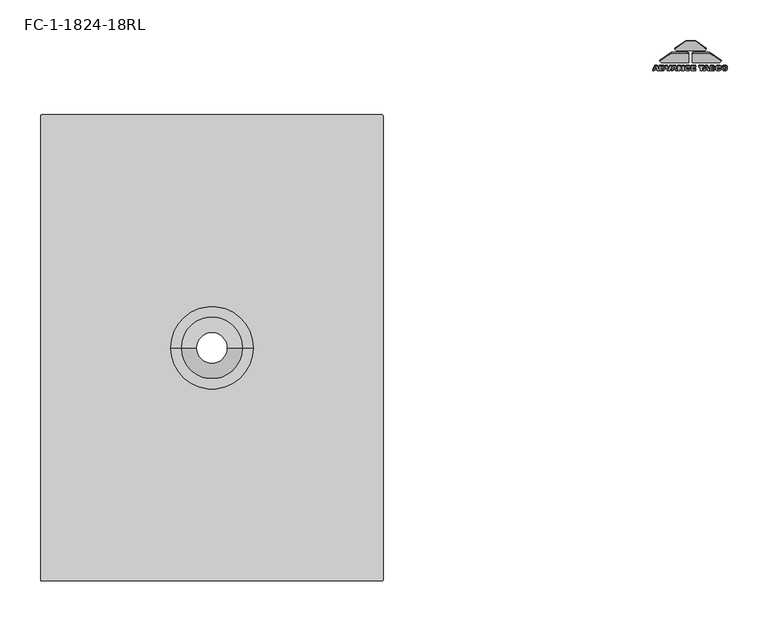
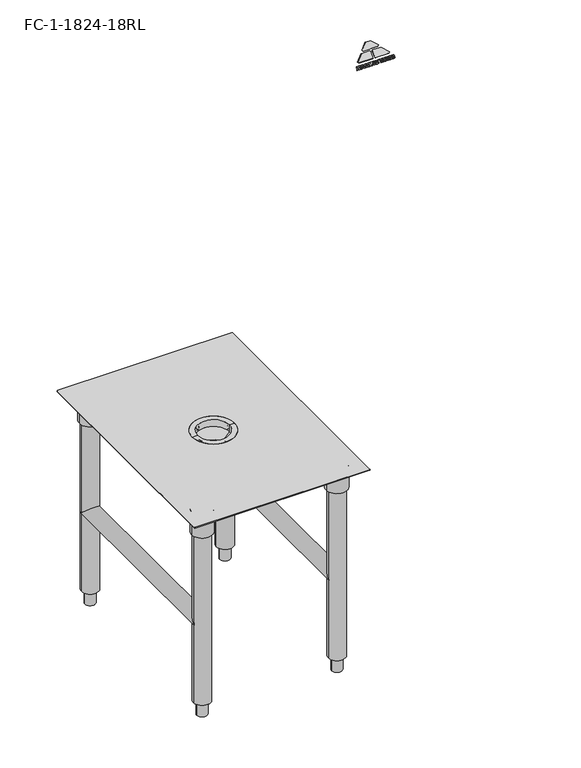
"""IFC4 building model written with IfcOpenShell, lengths in millimetres: proxy geometry, qf_advance_fc-1$2014$FC-1-1824-18RL : FC-1-1824-18RL."""

from ifc_helpers import new_model, si_unit, point, frame, frame_2d, origin, origin_with_axes, place, context, project, spatial, polyline, circle_curve, trimmed, segment, composite_curve, outline, extrude, source, transform, mapped, element, save
from ifc_brep_helpers import plane_surface, cylinder_surface, revolved_surface, advanced_brep


def fc_1_1824_18rl_d9c02636(model_context):
    return source(origin(), model_context, "Body", "SolidModel", [
        extrude(outline(polyline([(0.0, 0.0), (0.8986382, -2.992169), (-5.7928564, -7.4682591), (-6.3992546, -5.4491532), (-5.2268421, -4.6727099), (-6.0231962, -2.021113), (-7.4220948, -2.0434324), (-8.0357989, 0.0), (0.0, 0.0)]), holes=[polyline([(-1.0236432, -1.9782405), (-4.4880528, -2.0109168), (-3.9335816, -3.857123), (-1.0236432, -1.9782405)])]), frame((1231.0364, -35.8439941, 1043.6560059), z_axis=(0.0, -0.7071067811865482, 0.7071067811865468), x_axis=(0.28763785914895384, 0.6772239149587841, 0.6772239149587854)), (0.0, 0.0, 1.0), 1.5875),
        extrude(outline(composite_curve([segment(polyline([(1.7388284, -5.7897253), (2.9132681, -9.7002225)]), True, "CONTINUOUS"), segment(trimmed(circle_curve(frame_2d((0.4258756, -10.4472612)), 2.59715), [point((2.9132681, -9.7002225))], [point((1.1729143, -12.9346537))], False, "CARTESIAN"), True, "CONTINUOUS"), segment(polyline([(1.1729143, -12.9346537), (-1.2232536, -13.6542948)]), True, "CONTINUOUS"), segment(trimmed(circle_curve(frame_2d((-1.9702922, -11.1669024)), 2.59715), [point((-1.2232536, -13.6542948))], [point((-4.4576846, -11.913941))], False, "CARTESIAN"), True, "CONTINUOUS"), segment(polyline([(-4.4576846, -11.913941), (-5.6321244, -8.0034438), (1.7388284, -5.7897253)]), True, "CONTINUOUS")], self_intersect=False), holes=[composite_curve([segment(polyline([(-3.3131514, -9.4551704), (-2.7304978, -11.3952149)]), True, "CONTINUOUS"), segment(trimmed(circle_curve(frame_2d((-1.9702922, -11.1669024)), 0.79375), [point((-2.7304978, -11.3952149))], [point((-1.7419797, -11.9271079))], True, "CARTESIAN"), True, "CONTINUOUS"), segment(polyline([(-1.7419797, -11.9271079), (0.6541882, -11.2074667)]), True, "CONTINUOUS"), segment(trimmed(circle_curve(frame_2d((0.4258756, -10.4472612)), 0.79375), [point((0.6541882, -11.2074667))], [point((1.1860812, -10.2189486))], True, "CARTESIAN"), True, "CONTINUOUS"), segment(polyline([(1.1860812, -10.2189486), (0.6034275, -8.2789041), (-3.3131514, -9.4551704)]), True, "CONTINUOUS")], self_intersect=False)]), frame((1231.0364, -35.8439941, 1043.6560059), z_axis=(0.0, -0.7071067811865482, 0.7071067811865468), x_axis=(0.28763785914895384, 0.6772239149587841, 0.6772239149587854)), (0.0, 0.0, 1.0), 1.5875),
        extrude(outline(polyline([(3.8502629, -12.820106), (4.449355, -14.8148853), (-0.7608679, -18.1300438), (5.4356652, -18.0989732), (6.0493693, -20.1424056), (-1.9718176, -20.1910588), (-2.8923738, -17.1259101), (3.8502629, -12.820106)])), frame((1231.0364, -35.8439941, 1043.6560059), z_axis=(0.0, -0.7071067811865482, 0.7071067811865468), x_axis=(0.28763785914895384, 0.6772239149587841, 0.6772239149587854)), (0.0, 0.0, 1.0), 1.5875),
        extrude(outline(polyline([(-0.8905293, -23.7913921), (-1.5042335, -21.7479597), (6.5315655, -21.7479597), (7.4302036, -24.7401286), (0.738709, -29.2162188), (0.1323109, -27.1971129), (1.3047234, -26.4206696), (0.5083692, -23.7690727), (-0.8905293, -23.7913921)]), holes=[polyline([(2.0435127, -23.7588764), (2.5979839, -25.6050827), (5.5079223, -23.7262001), (2.0435127, -23.7588764)])]), frame((1231.0364, -35.8439941, 1043.6560059), z_axis=(0.0, -0.7071067811865482, 0.7071067811865468), x_axis=(0.28763785914895384, 0.6772239149587841, 0.6772239149587854)), (0.0, 0.0, 1.0), 1.5875),
        extrude(outline(polyline([(0.8994411, -29.7514035), (8.2703938, -27.537685), (9.2640101, -30.8460994), (4.2655808, -34.6015449), (9.8850202, -32.9138585), (10.4768063, -34.8843112), (3.1058536, -37.0980297), (2.0976253, -33.7409621), (7.1447075, -29.9709047), (1.4766152, -31.673203), (0.8994411, -29.7514035)])), frame((1231.0364, -35.8439941, 1043.6560059), z_axis=(0.0, -0.7071067811865482, 0.7071067811865468), x_axis=(0.28763785914895384, 0.6772239149587841, 0.6772239149587854)), (0.0, 0.0, 1.0), 1.5875),
        extrude(outline(composite_curve([segment(polyline([(10.2323563, -43.0996089), (9.7136302, -41.372422)]), True, "CONTINUOUS"), segment(trimmed(circle_curve(frame_2d((9.4853176, -40.6122165)), 0.79375), [point((9.7136302, -41.372422))], [point((10.2455232, -40.3839039))], True, "CARTESIAN"), True, "CONTINUOUS"), segment(polyline([(10.2455232, -40.3839039), (9.7888981, -38.8634929)]), True, "CONTINUOUS"), segment(trimmed(circle_curve(frame_2d((9.0286925, -39.0918054)), 0.79375), [point((9.7888981, -38.8634929))], [point((8.80038, -38.3315999))], True, "CARTESIAN"), True, "CONTINUOUS"), segment(polyline([(8.80038, -38.3315999), (6.4042121, -39.0512411)]), True, "CONTINUOUS"), segment(trimmed(circle_curve(frame_2d((6.6325247, -39.8114466)), 0.79375), [point((6.4042121, -39.0512411))], [point((5.8723192, -40.0397591))], True, "CARTESIAN"), True, "CONTINUOUS"), segment(polyline([(5.8723192, -40.0397591), (6.3289443, -41.5601702)]), True, "CONTINUOUS"), segment(trimmed(circle_curve(frame_2d((7.0891498, -41.3318576)), 0.79375), [point((6.3289443, -41.5601702))], [point((7.3174623, -42.0920632))], True, "CARTESIAN"), True, "CONTINUOUS"), segment(polyline([(7.3174623, -42.0920632), (7.8361884, -43.8192501)]), True, "CONTINUOUS"), segment(trimmed(circle_curve(frame_2d((7.0891498, -41.3318576)), 2.59715), [point((7.8361884, -43.8192501))], [point((4.6017574, -42.0788963))], False, "CARTESIAN"), True, "CONTINUOUS"), segment(polyline([(4.6017574, -42.0788963), (4.1451323, -40.5584852)]), True, "CONTINUOUS"), segment(trimmed(circle_curve(frame_2d((6.6325247, -39.8114466)), 2.59715), [point((4.1451323, -40.5584852))], [point((5.885486, -37.3240541))], False, "CARTESIAN"), True, "CONTINUOUS"), segment(polyline([(5.885486, -37.3240541), (8.2816539, -36.6044129)]), True, "CONTINUOUS"), segment(trimmed(circle_curve(frame_2d((9.0286925, -39.0918054)), 2.59715), [point((8.2816539, -36.6044129))], [point((11.5160851, -38.3447667))], False, "CARTESIAN"), True, "CONTINUOUS"), segment(polyline([(11.5160851, -38.3447667), (11.9727102, -39.8651778)]), True, "CONTINUOUS"), segment(trimmed(circle_curve(frame_2d((9.4853176, -40.6122165)), 2.59715), [point((11.9727102, -39.8651778))], [point((10.2323563, -43.0996089))], False, "CARTESIAN"), True, "CONTINUOUS")], self_intersect=False)), frame((1231.0364, -35.8439941, 1043.6560059), z_axis=(0.0, -0.7071067811865482, 0.7071067811865468), x_axis=(0.28763785914895384, 0.6772239149587841, 0.6772239149587854)), (0.0, 0.0, 1.0), 1.5875),
        extrude(outline(polyline([(12.9681529, -43.1796739), (14.5681672, -48.5071942), (12.9382866, -48.9966963), (11.9300584, -45.6396287), (10.6164232, -46.0341528), (11.5588974, -49.1722812), (10.1722825, -49.5887233), (9.2298083, -46.4505949), (7.8431934, -46.867037), (8.8733397, -50.2970843), (7.2191325, -50.7938924), (5.5972001, -45.3933924), (12.9681529, -43.1796739)])), frame((1231.0364, -35.8439941, 1043.6560059), z_axis=(0.0, -0.7071067811865482, 0.7071067811865468), x_axis=(0.28763785914895384, 0.6772239149587841, 0.6772239149587854)), (0.0, 0.0, 1.0), 1.5875),
        extrude(outline(polyline([(15.6567615, -52.1318541), (17.4102019, -57.9702326), (15.7073414, -58.4816527), (15.1155553, -56.5112), (9.447463, -58.2134984), (8.8556768, -56.2430456), (14.5237692, -54.5407473), (13.953901, -52.6432743), (15.6567615, -52.1318541)])), frame((1231.0364, -35.8439941, 1043.6560059), z_axis=(0.0, -0.7071067811865482, 0.7071067811865468), x_axis=(0.28763785914895384, 0.6772239149587841, 0.6772239149587854)), (0.0, 0.0, 1.0), 1.5875),
        extrude(outline(polyline([(9.9077411, -59.7460727), (17.94354, -59.7460727), (18.8421782, -62.7382416), (12.1506836, -67.2143318), (11.5442854, -65.1952259), (12.7166979, -64.4187826), (11.9203437, -61.7671857), (10.5214452, -61.7895051), (9.9077411, -59.7460727)]), holes=[polyline([(14.0099584, -63.6031957), (16.9198968, -61.7243132), (13.4554872, -61.7569894), (14.0099584, -63.6031957)])]), frame((1231.0364, -35.8439941, 1043.6560059), z_axis=(0.0, -0.7071067811865482, 0.7071067811865468), x_axis=(0.28763785914895384, 0.6772239149587841, 0.6772239149587854)), (0.0, 0.0, 1.0), 1.5875),
        extrude(outline(composite_curve([segment(polyline([(19.6750624, -65.5114714), (20.8732466, -69.50103)]), True, "CONTINUOUS"), segment(trimmed(circle_curve(frame_2d((18.9043499, -69.6343934)), 1.9734082), [point((20.8732466, -69.50103))], [point((17.1877703, -70.6078892))], False, "CARTESIAN"), True, "CONTINUOUS"), segment(trimmed(circle_curve(frame_2d((15.3204157, -71.0793546)), 1.9259524), [point((17.1877703, -70.6078892))], [point((13.4530612, -71.5508198))], False, "CARTESIAN"), True, "CONTINUOUS"), segment(polyline([(13.4530612, -71.5508198), (12.3041096, -67.7251899), (19.6750624, -65.5114714)]), True, "CONTINUOUS")], self_intersect=False), holes=[composite_curve([segment(polyline([(15.6697513, -68.8625705), (14.1644846, -69.3146473), (14.7343527, -71.2121203)]), True, "CONTINUOUS"), segment(trimmed(circle_curve(frame_2d((15.389333, -70.7098113)), 0.8254172), [point((14.7343527, -71.2121203))], [point((16.2133035, -70.6609635))], True, "CARTESIAN"), True, "CONTINUOUS"), segment(polyline([(16.2133035, -70.6609635), (15.6697513, -68.8625705)]), True, "CONTINUOUS")], self_intersect=False), composite_curve([segment(polyline([(18.8038562, -67.9213047), (17.3233327, -68.3659503), (17.8128348, -69.995831)]), True, "CONTINUOUS"), segment(trimmed(circle_curve(frame_2d((18.4548879, -69.4790507)), 0.824193), [point((17.8128348, -69.995831))], [point((19.2787463, -69.5025322))], True, "CARTESIAN"), True, "CONTINUOUS"), segment(polyline([(19.2787463, -69.5025322), (18.8038562, -67.9213047)]), True, "CONTINUOUS")], self_intersect=False)]), frame((1231.0364, -35.8439941, 1043.6560059), z_axis=(0.0, -0.7071067811865482, 0.7071067811865468), x_axis=(0.28763785914895384, 0.6772239149587841, 0.6772239149587854)), (0.0, 0.0, 1.0), 1.5875),
        extrude(outline(composite_curve([segment(trimmed(circle_curve(frame_2d((20.3799312, -76.8876879)), 2.59715), [point((22.8673237, -76.1406493))], [point((21.1269699, -79.3750804))], False, "CARTESIAN"), True, "CONTINUOUS"), segment(polyline([(21.1269699, -79.3750804), (20.6082437, -77.6478935)]), True, "CONTINUOUS"), segment(trimmed(circle_curve(frame_2d((20.3799312, -76.8876879)), 0.79375), [point((20.6082437, -77.6478935))], [point((21.1401367, -76.6593754))], True, "CARTESIAN"), True, "CONTINUOUS"), segment(polyline([(21.1401367, -76.6593754), (20.6835116, -75.1389643)]), True, "CONTINUOUS"), segment(trimmed(circle_curve(frame_2d((19.9233061, -75.3672769)), 0.79375), [point((20.6835116, -75.1389643))], [point((19.6949935, -74.6070714))], True, "CARTESIAN"), True, "CONTINUOUS"), segment(polyline([(19.6949935, -74.6070714), (17.2988257, -75.3267125)]), True, "CONTINUOUS"), segment(trimmed(circle_curve(frame_2d((17.5271382, -76.0869181)), 0.79375), [point((17.2988257, -75.3267125))], [point((16.7669327, -76.3152306))], True, "CARTESIAN"), True, "CONTINUOUS"), segment(polyline([(16.7669327, -76.3152306), (17.2235578, -77.8356417)]), True, "CONTINUOUS"), segment(trimmed(circle_curve(frame_2d((17.9837633, -77.6073291)), 0.79375), [point((17.2235578, -77.8356417))], [point((18.2120759, -78.3675346))], True, "CARTESIAN"), True, "CONTINUOUS"), segment(polyline([(18.2120759, -78.3675346), (18.730802, -80.0947216)]), True, "CONTINUOUS"), segment(trimmed(circle_curve(frame_2d((17.9837633, -77.6073291)), 2.59715), [point((18.730802, -80.0947216))], [point((15.4963709, -78.3543678))], False, "CARTESIAN"), True, "CONTINUOUS"), segment(polyline([(15.4963709, -78.3543678), (15.0397458, -76.8339567)]), True, "CONTINUOUS"), segment(trimmed(circle_curve(frame_2d((17.5271382, -76.0869181)), 2.59715), [point((15.0397458, -76.8339567))], [point((16.7800995, -73.5995256))], False, "CARTESIAN"), True, "CONTINUOUS"), segment(polyline([(16.7800995, -73.5995256), (19.1762674, -72.8798844)]), True, "CONTINUOUS"), segment(trimmed(circle_curve(frame_2d((19.9233061, -75.3672769)), 2.59715), [point((19.1762674, -72.8798844))], [point((22.4106986, -74.6202382))], False, "CARTESIAN"), True, "CONTINUOUS"), segment(polyline([(22.4106986, -74.6202382), (22.8673237, -76.1406493)]), True, "CONTINUOUS")], self_intersect=False)), frame((1231.0364, -35.8439941, 1043.6560059), z_axis=(0.0, -0.7071067811865482, 0.7071067811865468), x_axis=(0.28763785914895384, 0.6772239149587841, 0.6772239149587854)), (0.0, 0.0, 1.0), 1.5875),
        extrude(outline(composite_curve([segment(polyline([(18.9878987, -80.9507689), (21.3840666, -80.2311277)]), True, "CONTINUOUS"), segment(trimmed(circle_curve(frame_2d((22.1311052, -82.7185202)), 2.59715), [point((21.3840666, -80.2311277))], [point((24.6184977, -81.9714815))], False, "CARTESIAN"), True, "CONTINUOUS"), segment(polyline([(24.6184977, -81.9714815), (25.0751228, -83.4918925)]), True, "CONTINUOUS"), segment(trimmed(circle_curve(frame_2d((22.5877303, -84.2389312)), 2.59715), [point((25.0751228, -83.4918925))], [point((23.1187153, -86.7812222))], False, "CARTESIAN"), True, "CONTINUOUS"), segment(polyline([(23.1187153, -86.7812222), (20.7225475, -87.5008633)]), True, "CONTINUOUS"), segment(trimmed(circle_curve(frame_2d((20.1915625, -84.9585724)), 2.59715), [point((20.7225475, -87.5008633))], [point((17.7041701, -85.705611))], False, "CARTESIAN"), True, "CONTINUOUS"), segment(polyline([(17.7041701, -85.705611), (17.247545, -84.1852)]), True, "CONTINUOUS"), segment(trimmed(circle_curve(frame_2d((19.7349374, -83.4381613)), 2.59715), [point((17.247545, -84.1852))], [point((18.9878987, -80.9507689))], False, "CARTESIAN"), True, "CONTINUOUS")], self_intersect=False), holes=[composite_curve([segment(polyline([(18.9747318, -83.6664739), (19.4313569, -85.1868849)]), True, "CONTINUOUS"), segment(trimmed(circle_curve(frame_2d((20.1915625, -84.9585724)), 0.79375), [point((19.4313569, -85.1868849))], [point((20.2994506, -85.7449561))], True, "CARTESIAN"), True, "CONTINUOUS"), segment(polyline([(20.2994506, -85.7449561), (22.6956183, -85.0253149)]), True, "CONTINUOUS"), segment(trimmed(circle_curve(frame_2d((22.5877303, -84.2389312)), 0.79375), [point((22.6956183, -85.0253149))], [point((23.3479358, -84.0106187))], True, "CARTESIAN"), True, "CONTINUOUS"), segment(polyline([(23.3479358, -84.0106187), (22.8913107, -82.4902076)]), True, "CONTINUOUS"), segment(trimmed(circle_curve(frame_2d((22.1311052, -82.7185202)), 0.79375), [point((22.8913107, -82.4902076))], [point((21.9027927, -81.9583146))], True, "CARTESIAN"), True, "CONTINUOUS"), segment(polyline([(21.9027927, -81.9583146), (19.5066248, -82.6779558)]), True, "CONTINUOUS"), segment(trimmed(circle_curve(frame_2d((19.7349374, -83.4381613)), 0.79375), [point((19.5066248, -82.6779558))], [point((18.9747318, -83.6664739))], True, "CARTESIAN"), True, "CONTINUOUS")], self_intersect=False)]), frame((1231.0364, -35.8439941, 1043.6560059), z_axis=(0.0, -0.7071067811865482, 0.7071067811865468), x_axis=(0.28763785914895384, 0.6772239149587841, 0.6772239149587854)), (0.0, 0.0, 1.0), 1.5875),
        extrude(outline(polyline([(55.8503682, -36.1089094), (46.7199535, -52.7744612), (43.69559, -51.7997924), (33.5402477, -17.9858506), (35.527159, -15.5061455), (52.3580994, -24.4808057), (55.8503682, -36.1089094)])), frame((1231.0364, -35.8439941, 1043.6560059), z_axis=(0.0, -0.7071067811865482, 0.7071067811865468), x_axis=(0.28763785914895384, 0.6772239149587841, 0.6772239149587854)), (0.0, 0.0, 1.0), 1.5875),
        extrude(outline(polyline([(41.641881, -58.6489682), (31.7210534, -76.2149243), (28.8426493, -75.1964196), (19.1621971, -42.9637053), (34.1473684, -38.4632083), (35.8189977, -39.2606864), (41.641881, -58.6489682)])), frame((1231.0364, -35.8439941, 1043.6560059), z_axis=(0.0, -0.7071067811865482, 0.7071067811865468), x_axis=(0.28763785914895384, 0.6772239149587841, 0.6772239149587854)), (0.0, 0.0, 1.0), 1.5875),
        extrude(outline(polyline([(27.9285159, -12.9879835), (33.7513992, -32.3762652), (32.7957581, -33.9627916), (17.8105868, -38.4632885), (8.1301347, -6.2305742), (9.9710865, -3.7947051), (27.9285159, -12.9879835)])), frame((1231.0364, -35.8439941, 1043.6560059), z_axis=(0.0, -0.7071067811865482, 0.7071067811865468), x_axis=(0.28763785914895384, 0.6772239149587841, 0.6772239149587854)), (0.0, 0.0, 1.0), 1.5875),
        extrude(outline(composite_curve([segment(polyline([(233.3625, 502.8701209), (233.3625, 504.4576209)]), True, "CONTINUOUS"), segment(trimmed(circle_curve(frame_2d((233.3625, 523.5076209)), 19.05), [point((233.3625, 504.4576209))], [point((233.3625, 542.5576209))], True, "CARTESIAN"), True, "CONTINUOUS"), segment(polyline([(233.3625, 542.5576209), (233.3625, 544.1451209)]), True, "CONTINUOUS"), segment(trimmed(circle_curve(frame_2d((233.3625, 523.5076209)), 20.6375), [point((233.3625, 544.1451209))], [point((233.3625, 502.8701209))], False, "CARTESIAN"), True, "CONTINUOUS")], self_intersect=False)), frame((0.0, -619.7718402, 0.0), z_axis=(0.0, 1.0, 0.0), x_axis=(0.0, 0.0, 1.0)), (0.0, 0.0, 1.0), 469.9),
        extrude(outline(composite_curve([segment(trimmed(circle_curve(frame_2d((523.5071331, -150.8289041)), 12.7), [point((510.8071331, -150.8289041))], [point((536.2071331, -150.8289041))], False, "CARTESIAN"), True, "CONTINUOUS"), segment(trimmed(circle_curve(frame_2d((523.5071331, -150.8289041)), 12.7), [point((536.2071331, -150.8289041))], [point((510.8071331, -150.8289041))], False, "CARTESIAN"), True, "CONTINUOUS")], self_intersect=False)), origin_with_axes(), (0.0, 0.0, 1.0), 34.925),
        extrude(outline(composite_curve([segment(trimmed(circle_curve(frame_2d((523.5071331, -617.5210959)), 12.7), [point((510.8071331, -617.5210959))], [point((536.2071331, -617.5210959))], False, "CARTESIAN"), True, "CONTINUOUS"), segment(trimmed(circle_curve(frame_2d((523.5071331, -617.5210959)), 12.7), [point((536.2071331, -617.5210959))], [point((510.8071331, -617.5210959))], False, "CARTESIAN"), True, "CONTINUOUS")], self_intersect=False)), origin_with_axes(), (0.0, 0.0, 1.0), 34.925),
        extrude(outline(composite_curve([segment(trimmed(circle_curve(frame_2d((523.5071331, -150.8289041)), 20.6375), [point((502.8696331, -150.8289041))], [point((544.1446331, -150.8289041))], False, "CARTESIAN"), True, "CONTINUOUS"), segment(trimmed(circle_curve(frame_2d((523.5071331, -150.8289041)), 20.6375), [point((544.1446331, -150.8289041))], [point((502.8696331, -150.8289041))], False, "CARTESIAN"), True, "CONTINUOUS")], self_intersect=False)), frame((0.0, 0.0, 34.925), z_axis=(0.0, 0.0, 1.0), x_axis=(1.0, 0.0, 0.0)), (0.0, 0.0, 1.0), 428.617356),
        extrude(outline(composite_curve([segment(trimmed(circle_curve(frame_2d((523.5071331, -617.5210959)), 20.6375), [point((502.8696331, -617.5210959))], [point((544.1446331, -617.5210959))], False, "CARTESIAN"), True, "CONTINUOUS"), segment(trimmed(circle_curve(frame_2d((523.5071331, -617.5210959)), 20.6375), [point((544.1446331, -617.5210959))], [point((502.8696331, -617.5210959))], False, "CARTESIAN"), True, "CONTINUOUS")], self_intersect=False)), frame((0.0, 0.0, 34.925), z_axis=(0.0, 0.0, 1.0), x_axis=(1.0, 0.0, 0.0)), (0.0, 0.0, 1.0), 428.617356),
        extrude(outline(composite_curve([segment(trimmed(circle_curve(frame_2d((523.5071331, -150.8319462)), 25.4), [point((498.1071331, -150.8319462))], [point((548.9071331, -150.8319462))], False, "CARTESIAN"), True, "CONTINUOUS"), segment(trimmed(circle_curve(frame_2d((523.5071331, -150.8319462)), 25.4), [point((548.9071331, -150.8319462))], [point((498.1071331, -150.8319462))], False, "CARTESIAN"), True, "CONTINUOUS")], self_intersect=False)), frame((0.0, 0.0, 463.542356), z_axis=(0.0, 0.0, 1.0), x_axis=(1.0, 0.0, 0.0)), (0.0, 0.0, 1.0), 57.15),
        extrude(outline(composite_curve([segment(trimmed(circle_curve(frame_2d((523.5071331, -617.5180538)), 25.4), [point((498.1071331, -617.5180538))], [point((548.9071331, -617.5180538))], False, "CARTESIAN"), True, "CONTINUOUS"), segment(trimmed(circle_curve(frame_2d((523.5071331, -617.5180538)), 25.4), [point((548.9071331, -617.5180538))], [point((498.1071331, -617.5180538))], False, "CARTESIAN"), True, "CONTINUOUS")], self_intersect=False)), frame((0.0, 0.0, 463.542356), z_axis=(0.0, 0.0, 1.0), x_axis=(1.0, 0.0, 0.0)), (0.0, 0.0, 1.0), 57.15),
        extrude(outline(composite_curve([segment(trimmed(circle_curve(frame_2d((233.3625, 848.0923791)), 20.6375), [point((233.3625, 868.7298791))], [point((233.3625, 827.4548791))], False, "CARTESIAN"), True, "CONTINUOUS"), segment(polyline([(233.3625, 827.4548791), (233.3625, 829.0423791)]), True, "CONTINUOUS"), segment(trimmed(circle_curve(frame_2d((233.3625, 848.0923791)), 19.05), [point((233.3625, 829.0423791))], [point((233.3625, 867.1423791))], True, "CARTESIAN"), True, "CONTINUOUS"), segment(polyline([(233.3625, 867.1423791), (233.3625, 868.7298791)]), True, "CONTINUOUS")], self_intersect=False)), frame((0.0, -619.7718402, 0.0), z_axis=(0.0, 1.0, 0.0), x_axis=(0.0, 0.0, 1.0)), (0.0, 0.0, 1.0), 469.9),
        extrude(outline(composite_curve([segment(trimmed(circle_curve(frame_2d((848.0928669, -150.8289041)), 12.7), [point((860.7928669, -150.8289041))], [point((835.3928669, -150.8289041))], False, "CARTESIAN"), True, "CONTINUOUS"), segment(trimmed(circle_curve(frame_2d((848.0928669, -150.8289041)), 12.7), [point((835.3928669, -150.8289041))], [point((860.7928669, -150.8289041))], False, "CARTESIAN"), True, "CONTINUOUS")], self_intersect=False)), origin_with_axes(), (0.0, 0.0, 1.0), 34.925),
        extrude(outline(composite_curve([segment(trimmed(circle_curve(frame_2d((848.0928669, -617.5210959)), 12.7), [point((860.7928669, -617.5210959))], [point((835.3928669, -617.5210959))], False, "CARTESIAN"), True, "CONTINUOUS"), segment(trimmed(circle_curve(frame_2d((848.0928669, -617.5210959)), 12.7), [point((835.3928669, -617.5210959))], [point((860.7928669, -617.5210959))], False, "CARTESIAN"), True, "CONTINUOUS")], self_intersect=False)), origin_with_axes(), (0.0, 0.0, 1.0), 34.925),
        extrude(outline(composite_curve([segment(trimmed(circle_curve(frame_2d((848.0928669, -150.8289041)), 20.6375), [point((868.7303669, -150.8289041))], [point((827.4553669, -150.8289041))], False, "CARTESIAN"), True, "CONTINUOUS"), segment(trimmed(circle_curve(frame_2d((848.0928669, -150.8289041)), 20.6375), [point((827.4553669, -150.8289041))], [point((868.7303669, -150.8289041))], False, "CARTESIAN"), True, "CONTINUOUS")], self_intersect=False)), frame((0.0, 0.0, 34.925), z_axis=(0.0, 0.0, 1.0), x_axis=(1.0, 0.0, 0.0)), (0.0, 0.0, 1.0), 428.617356),
        extrude(outline(composite_curve([segment(trimmed(circle_curve(frame_2d((848.0928669, -617.5210959)), 20.6375), [point((868.7303669, -617.5210959))], [point((827.4553669, -617.5210959))], False, "CARTESIAN"), True, "CONTINUOUS"), segment(trimmed(circle_curve(frame_2d((848.0928669, -617.5210959)), 20.6375), [point((827.4553669, -617.5210959))], [point((868.7303669, -617.5210959))], False, "CARTESIAN"), True, "CONTINUOUS")], self_intersect=False)), frame((0.0, 0.0, 34.925), z_axis=(0.0, 0.0, 1.0), x_axis=(1.0, 0.0, 0.0)), (0.0, 0.0, 1.0), 428.617356),
        extrude(outline(composite_curve([segment(trimmed(circle_curve(frame_2d((848.0928669, -150.8319462)), 25.4), [point((873.4928669, -150.8319462))], [point((822.6928669, -150.8319462))], False, "CARTESIAN"), True, "CONTINUOUS"), segment(trimmed(circle_curve(frame_2d((848.0928669, -150.8319462)), 25.4), [point((822.6928669, -150.8319462))], [point((873.4928669, -150.8319462))], False, "CARTESIAN"), True, "CONTINUOUS")], self_intersect=False)), frame((0.0, 0.0, 463.542356), z_axis=(0.0, 0.0, 1.0), x_axis=(1.0, 0.0, 0.0)), (0.0, 0.0, 1.0), 57.15),
        extrude(outline(composite_curve([segment(trimmed(circle_curve(frame_2d((848.0928669, -617.5180538)), 25.4), [point((873.4928669, -617.5180538))], [point((822.6928669, -617.5180538))], False, "CARTESIAN"), True, "CONTINUOUS"), segment(trimmed(circle_curve(frame_2d((848.0928669, -617.5180538)), 25.4), [point((822.6928669, -617.5180538))], [point((873.4928669, -617.5180538))], False, "CARTESIAN"), True, "CONTINUOUS")], self_intersect=False)), frame((0.0, 0.0, 463.542356), z_axis=(0.0, 0.0, 1.0), x_axis=(1.0, 0.0, 0.0)), (0.0, 0.0, 1.0), 57.15),
        advanced_brep(
        [(723.9, -384.175, 504.8173689), (647.7, -384.175, 504.8173689), (666.75, -384.175, 484.1798689), (704.85, -384.175, 484.1798689), (723.9, -384.175, 522.2798689), (647.7, -384.175, 522.2798689), (736.6, -384.175, 522.2798689), (635.0, -384.175, 522.2798689), (736.6, -384.175, 520.6923689), (635.0, -384.175, 520.6923689), (725.4875, -384.175, 520.6923689), (646.1125, -384.175, 520.6923689), (725.4875, -384.175, 517.638172), (646.1125, -384.175, 517.638172), (726.6076242, -384.175, 516.5180479), (644.9923758, -384.175, 516.5180479), (725.4875, -384.175, 515.3979237), (646.1125, -384.175, 515.3979237), (726.6076242, -384.175, 514.2777995), (644.9923758, -384.175, 514.2777995), (725.4875, -384.175, 513.1576754), (646.1125, -384.175, 513.1576754), (726.6076242, -384.175, 512.0375512), (644.9923758, -384.175, 512.0375512), (725.4875, -384.175, 510.9174271), (646.1125, -384.175, 510.9174271), (726.6076242, -384.175, 509.7973029), (644.9923758, -384.175, 509.7973029), (725.4875, -384.175, 508.6771787), (646.1125, -384.175, 508.6771787), (726.6076242, -384.175, 507.5570546), (644.9923758, -384.175, 507.5570546), (725.4875, -384.175, 506.4369304), (646.1125, -384.175, 506.4369304), (726.6076242, -384.175, 505.3168062), (644.9923758, -384.175, 505.3168062), (725.4875, -384.175, 504.1966821), (646.1125, -384.175, 504.1966821), (706.4375, -384.175, 483.5591821), (665.1625, -384.175, 483.5591821), (706.4375, -384.175, 481.0936105), (665.1625, -384.175, 481.0936105), (707.5576242, -384.175, 479.9734864), (664.0423758, -384.175, 479.9734864), (706.4375, -384.175, 478.8533622), (665.1625, -384.175, 478.8533622), (707.5576242, -384.175, 477.733238), (664.0423758, -384.175, 477.733238), (706.4375, -384.175, 476.6131139), (665.1625, -384.175, 476.6131139), (707.5576242, -384.175, 475.4929897), (664.0423758, -384.175, 475.4929897), (706.4375, -384.175, 474.3728656), (665.1625, -384.175, 474.3728656), (707.5576242, -384.175, 473.2527414), (664.0423758, -384.175, 473.2527414), (706.4375, -384.175, 472.1326172), (665.1625, -384.175, 472.1326172), (707.5576242, -384.175, 471.0124931), (664.0423758, -384.175, 471.0124931), (706.4375, -384.175, 469.8923689), (665.1625, -384.175, 469.8923689), (704.85, -384.175, 469.8923689), (666.75, -384.175, 469.8923689)],
        [
            (0, 1, circle_curve(frame((685.8, -384.175, 504.8173689), z_axis=(0.0, 0.0, 1.0), x_axis=(-1.0, 0.0, 0.0)), 38.1)),
            (1, 2),
            (2, 3, circle_curve(frame((685.8, -384.175, 484.1798689), z_axis=(0.0, 0.0, -1.0), x_axis=(-1.0, 0.0, 0.0)), 19.05)),
            (3, 0),
            (1, 0, circle_curve(frame((685.8, -384.175, 504.8173689), z_axis=(0.0, 0.0, 1.0), x_axis=(-1.0, 0.0, 0.0)), 38.1)),
            (3, 2, circle_curve(frame((685.8, -384.175, 484.1798689), z_axis=(0.0, 0.0, -1.0), x_axis=(-1.0, 0.0, 0.0)), 19.05)),
            (4, 5, circle_curve(frame((685.8, -384.175, 522.2798689), z_axis=(0.0, 0.0, 1.0), x_axis=(-1.0, 0.0, 0.0)), 38.1)),
            (5, 1),
            (0, 4),
            (5, 4, circle_curve(frame((685.8, -384.175, 522.2798689), z_axis=(0.0, 0.0, 1.0), x_axis=(-1.0, 0.0, 0.0)), 38.1)),
            (6, 7, circle_curve(frame((685.8, -384.175, 522.2798689), z_axis=(0.0, 0.0, 1.0), x_axis=(-1.0, 0.0, 0.0)), 50.8)),
            (7, 5),
            (4, 6),
            (7, 6, circle_curve(frame((685.8, -384.175, 522.2798689), z_axis=(0.0, 0.0, 1.0), x_axis=(-1.0, 0.0, 0.0)), 50.8)),
            (8, 9, circle_curve(frame((685.8, -384.175, 520.6923689), z_axis=(0.0, 0.0, 1.0), x_axis=(-1.0, 0.0, 0.0)), 50.8)),
            (9, 7),
            (6, 8),
            (9, 8, circle_curve(frame((685.8, -384.175, 520.6923689), z_axis=(0.0, 0.0, 1.0), x_axis=(-1.0, 0.0, 0.0)), 50.8)),
            (10, 11, circle_curve(frame((685.8, -384.175, 520.6923689), z_axis=(0.0, 0.0, 1.0), x_axis=(-1.0, 0.0, 0.0)), 39.6875)),
            (11, 9),
            (8, 10),
            (11, 10, circle_curve(frame((685.8, -384.175, 520.6923689), z_axis=(0.0, 0.0, 1.0), x_axis=(-1.0, 0.0, 0.0)), 39.6875)),
            (12, 13, circle_curve(frame((685.8, -384.175, 517.638172), z_axis=(0.0, 0.0, 1.0), x_axis=(-1.0, 0.0, 0.0)), 39.6875)),
            (13, 11),
            (10, 12),
            (13, 12, circle_curve(frame((685.8, -384.175, 517.638172), z_axis=(0.0, 0.0, 1.0), x_axis=(-1.0, 0.0, 0.0)), 39.6875)),
            (14, 15, circle_curve(frame((685.8, -384.175, 516.5180479), z_axis=(0.0, 0.0, 1.0), x_axis=(-1.0, 0.0, 0.0)), 40.8076242)),
            (15, 13),
            (12, 14),
            (15, 14, circle_curve(frame((685.8, -384.175, 516.5180479), z_axis=(0.0, 0.0, 1.0), x_axis=(-1.0, 0.0, 0.0)), 40.8076242)),
            (16, 17, circle_curve(frame((685.8, -384.175, 515.3979237), z_axis=(0.0, 0.0, 1.0), x_axis=(-1.0, 0.0, 0.0)), 39.6875)),
            (17, 15),
            (14, 16),
            (17, 16, circle_curve(frame((685.8, -384.175, 515.3979237), z_axis=(0.0, 0.0, 1.0), x_axis=(-1.0, 0.0, 0.0)), 39.6875)),
            (18, 19, circle_curve(frame((685.8, -384.175, 514.2777995), z_axis=(0.0, 0.0, 1.0), x_axis=(-1.0, 0.0, 0.0)), 40.8076242)),
            (19, 17),
            (16, 18),
            (19, 18, circle_curve(frame((685.8, -384.175, 514.2777995), z_axis=(0.0, 0.0, 1.0), x_axis=(-1.0, 0.0, 0.0)), 40.8076242)),
            (20, 21, circle_curve(frame((685.8, -384.175, 513.1576754), z_axis=(0.0, 0.0, 1.0), x_axis=(-1.0, 0.0, 0.0)), 39.6875)),
            (21, 19),
            (18, 20),
            (21, 20, circle_curve(frame((685.8, -384.175, 513.1576754), z_axis=(0.0, 0.0, 1.0), x_axis=(-1.0, 0.0, 0.0)), 39.6875)),
            (22, 23, circle_curve(frame((685.8, -384.175, 512.0375512), z_axis=(0.0, 0.0, 1.0), x_axis=(-1.0, 0.0, 0.0)), 40.8076242)),
            (23, 21),
            (20, 22),
            (23, 22, circle_curve(frame((685.8, -384.175, 512.0375512), z_axis=(0.0, 0.0, 1.0), x_axis=(-1.0, 0.0, 0.0)), 40.8076242)),
            (24, 25, circle_curve(frame((685.8, -384.175, 510.9174271), z_axis=(0.0, 0.0, 1.0), x_axis=(-1.0, 0.0, 0.0)), 39.6875)),
            (25, 23),
            (22, 24),
            (25, 24, circle_curve(frame((685.8, -384.175, 510.9174271), z_axis=(0.0, 0.0, 1.0), x_axis=(-1.0, 0.0, 0.0)), 39.6875)),
            (26, 27, circle_curve(frame((685.8, -384.175, 509.7973029), z_axis=(0.0, 0.0, 1.0), x_axis=(-1.0, 0.0, 0.0)), 40.8076242)),
            (27, 25),
            (24, 26),
            (27, 26, circle_curve(frame((685.8, -384.175, 509.7973029), z_axis=(0.0, 0.0, 1.0), x_axis=(-1.0, 0.0, 0.0)), 40.8076242)),
            (28, 29, circle_curve(frame((685.8, -384.175, 508.6771787), z_axis=(0.0, 0.0, 1.0), x_axis=(-1.0, 0.0, 0.0)), 39.6875)),
            (29, 27),
            (26, 28),
            (29, 28, circle_curve(frame((685.8, -384.175, 508.6771787), z_axis=(0.0, 0.0, 1.0), x_axis=(-1.0, 0.0, 0.0)), 39.6875)),
            (30, 31, circle_curve(frame((685.8, -384.175, 507.5570546), z_axis=(0.0, 0.0, 1.0), x_axis=(-1.0, 0.0, 0.0)), 40.8076242)),
            (31, 29),
            (28, 30),
            (31, 30, circle_curve(frame((685.8, -384.175, 507.5570546), z_axis=(0.0, 0.0, 1.0), x_axis=(-1.0, 0.0, 0.0)), 40.8076242)),
            (32, 33, circle_curve(frame((685.8, -384.175, 506.4369304), z_axis=(0.0, 0.0, 1.0), x_axis=(-1.0, 0.0, 0.0)), 39.6875)),
            (33, 31),
            (30, 32),
            (33, 32, circle_curve(frame((685.8, -384.175, 506.4369304), z_axis=(0.0, 0.0, 1.0), x_axis=(-1.0, 0.0, 0.0)), 39.6875)),
            (34, 35, circle_curve(frame((685.8, -384.175, 505.3168062), z_axis=(0.0, 0.0, 1.0), x_axis=(-1.0, 0.0, 0.0)), 40.8076242)),
            (35, 33),
            (32, 34),
            (35, 34, circle_curve(frame((685.8, -384.175, 505.3168062), z_axis=(0.0, 0.0, 1.0), x_axis=(-1.0, 0.0, 0.0)), 40.8076242)),
            (36, 37, circle_curve(frame((685.8, -384.175, 504.1966821), z_axis=(0.0, 0.0, 1.0), x_axis=(-1.0, 0.0, 0.0)), 39.6875)),
            (37, 35),
            (34, 36),
            (37, 36, circle_curve(frame((685.8, -384.175, 504.1966821), z_axis=(0.0, 0.0, 1.0), x_axis=(-1.0, 0.0, 0.0)), 39.6875)),
            (38, 39, circle_curve(frame((685.8, -384.175, 483.5591821), z_axis=(0.0, 0.0, 1.0), x_axis=(-1.0, 0.0, 0.0)), 20.6375)),
            (39, 37),
            (36, 38),
            (39, 38, circle_curve(frame((685.8, -384.175, 483.5591821), z_axis=(0.0, 0.0, 1.0), x_axis=(-1.0, 0.0, 0.0)), 20.6375)),
            (40, 41, circle_curve(frame((685.8, -384.175, 481.0936105), z_axis=(0.0, 0.0, 1.0), x_axis=(-1.0, 0.0, 0.0)), 20.6375)),
            (41, 39),
            (38, 40),
            (41, 40, circle_curve(frame((685.8, -384.175, 481.0936105), z_axis=(0.0, 0.0, 1.0), x_axis=(-1.0, 0.0, 0.0)), 20.6375)),
            (42, 43, circle_curve(frame((685.8, -384.175, 479.9734864), z_axis=(0.0, 0.0, 1.0), x_axis=(-1.0, 0.0, 0.0)), 21.7576242)),
            (43, 41),
            (40, 42),
            (43, 42, circle_curve(frame((685.8, -384.175, 479.9734864), z_axis=(0.0, 0.0, 1.0), x_axis=(-1.0, 0.0, 0.0)), 21.7576242)),
            (44, 45, circle_curve(frame((685.8, -384.175, 478.8533622), z_axis=(0.0, 0.0, 1.0), x_axis=(-1.0, 0.0, 0.0)), 20.6375)),
            (45, 43),
            (42, 44),
            (45, 44, circle_curve(frame((685.8, -384.175, 478.8533622), z_axis=(0.0, 0.0, 1.0), x_axis=(-1.0, 0.0, 0.0)), 20.6375)),
            (46, 47, circle_curve(frame((685.8, -384.175, 477.733238), z_axis=(0.0, 0.0, 1.0), x_axis=(-1.0, 0.0, 0.0)), 21.7576242)),
            (47, 45),
            (44, 46),
            (47, 46, circle_curve(frame((685.8, -384.175, 477.733238), z_axis=(0.0, 0.0, 1.0), x_axis=(-1.0, 0.0, 0.0)), 21.7576242)),
            (48, 49, circle_curve(frame((685.8, -384.175, 476.6131139), z_axis=(0.0, 0.0, 1.0), x_axis=(-1.0, 0.0, 0.0)), 20.6375)),
            (49, 47),
            (46, 48),
            (49, 48, circle_curve(frame((685.8, -384.175, 476.6131139), z_axis=(0.0, 0.0, 1.0), x_axis=(-1.0, 0.0, 0.0)), 20.6375)),
            (50, 51, circle_curve(frame((685.8, -384.175, 475.4929897), z_axis=(0.0, 0.0, 1.0), x_axis=(-1.0, 0.0, 0.0)), 21.7576242)),
            (51, 49),
            (48, 50),
            (51, 50, circle_curve(frame((685.8, -384.175, 475.4929897), z_axis=(0.0, 0.0, 1.0), x_axis=(-1.0, 0.0, 0.0)), 21.7576242)),
            (52, 53, circle_curve(frame((685.8, -384.175, 474.3728656), z_axis=(0.0, 0.0, 1.0), x_axis=(-1.0, 0.0, 0.0)), 20.6375)),
            (53, 51),
            (50, 52),
            (53, 52, circle_curve(frame((685.8, -384.175, 474.3728656), z_axis=(0.0, 0.0, 1.0), x_axis=(-1.0, 0.0, 0.0)), 20.6375)),
            (54, 55, circle_curve(frame((685.8, -384.175, 473.2527414), z_axis=(0.0, 0.0, 1.0), x_axis=(-1.0, 0.0, 0.0)), 21.7576242)),
            (55, 53),
            (52, 54),
            (55, 54, circle_curve(frame((685.8, -384.175, 473.2527414), z_axis=(0.0, 0.0, 1.0), x_axis=(-1.0, 0.0, 0.0)), 21.7576242)),
            (56, 57, circle_curve(frame((685.8, -384.175, 472.1326172), z_axis=(0.0, 0.0, 1.0), x_axis=(-1.0, 0.0, 0.0)), 20.6375)),
            (57, 55),
            (54, 56),
            (57, 56, circle_curve(frame((685.8, -384.175, 472.1326172), z_axis=(0.0, 0.0, 1.0), x_axis=(-1.0, 0.0, 0.0)), 20.6375)),
            (58, 59, circle_curve(frame((685.8, -384.175, 471.0124931), z_axis=(0.0, 0.0, 1.0), x_axis=(-1.0, 0.0, 0.0)), 21.7576242)),
            (59, 57),
            (56, 58),
            (59, 58, circle_curve(frame((685.8, -384.175, 471.0124931), z_axis=(0.0, 0.0, 1.0), x_axis=(-1.0, 0.0, 0.0)), 21.7576242)),
            (60, 61, circle_curve(frame((685.8, -384.175, 469.8923689), z_axis=(0.0, 0.0, 1.0), x_axis=(-1.0, 0.0, 0.0)), 20.6375)),
            (61, 59),
            (58, 60),
            (61, 60, circle_curve(frame((685.8, -384.175, 469.8923689), z_axis=(0.0, 0.0, 1.0), x_axis=(-1.0, 0.0, 0.0)), 20.6375)),
            (62, 63, circle_curve(frame((685.8, -384.175, 469.8923689), z_axis=(0.0, 0.0, 1.0), x_axis=(-1.0, 0.0, 0.0)), 19.05)),
            (63, 61),
            (60, 62),
            (63, 62, circle_curve(frame((685.8, -384.175, 469.8923689), z_axis=(0.0, 0.0, 1.0), x_axis=(-1.0, 0.0, 0.0)), 19.05)),
            (2, 63),
            (62, 3),
        ],
        [
            revolved_surface(polyline([(666.75, -384.175, 484.1798689), (647.7, -384.175, 504.8173689)]), (685.8, -384.175, -304.8), (0.0, 0.0, -1.0)),
            revolved_surface(polyline([(647.6999999999999, -384.175, 504.81736889999996), (647.6999999999999, -384.175, 522.2798689000001)]), (685.8, -384.175, -304.8), (0.0, 0.0, -1.0)),
            plane_surface(frame((685.8, -384.175, 522.2798689), z_axis=(0.0, 0.0, 1.0), x_axis=(-1.0, 0.0, 0.0))),
            cylinder_surface(frame((685.8, -384.175, -304.8), z_axis=(0.0, 0.0, -1.0), x_axis=(-1.0, 0.0, 0.0)), 50.8),
            plane_surface(frame((685.8, -384.175, 520.6923689), z_axis=(0.0, 0.0, -1.0), x_axis=(-1.0, 0.0, 0.0))),
            cylinder_surface(frame((685.8, -384.175, -304.8), z_axis=(0.0, 0.0, -1.0), x_axis=(-1.0, 0.0, 0.0)), 39.6875),
            revolved_surface(polyline([(646.1125, -384.175, 517.638172), (644.9923758, -384.175, 516.5180479)]), (685.8, -384.175, -304.8), (0.0, 0.0, -1.0)),
            revolved_surface(polyline([(644.9923758, -384.175, 516.5180479), (646.1125, -384.175, 515.3979237)]), (685.8, -384.175, -304.8), (0.0, 0.0, -1.0)),
            revolved_surface(polyline([(646.1125, -384.175, 515.3979237), (644.9923758, -384.175, 514.2777995)]), (685.8, -384.175, -304.8), (0.0, 0.0, -1.0)),
            revolved_surface(polyline([(644.9923758, -384.175, 514.2777995), (646.1125, -384.175, 513.1576754)]), (685.8, -384.175, -304.8), (0.0, 0.0, -1.0)),
            revolved_surface(polyline([(646.1125, -384.175, 513.1576754), (644.9923758, -384.175, 512.0375512)]), (685.8, -384.175, -304.8), (0.0, 0.0, -1.0)),
            revolved_surface(polyline([(644.9923758, -384.175, 512.0375512), (646.1125, -384.175, 510.9174271)]), (685.8, -384.175, -304.8), (0.0, 0.0, -1.0)),
            revolved_surface(polyline([(646.1125, -384.175, 510.9174271), (644.9923758, -384.175, 509.7973029)]), (685.8, -384.175, -304.8), (0.0, 0.0, -1.0)),
            revolved_surface(polyline([(644.9923758, -384.175, 509.7973029), (646.1125, -384.175, 508.6771787)]), (685.8, -384.175, -304.8), (0.0, 0.0, -1.0)),
            revolved_surface(polyline([(646.1125, -384.175, 508.6771787), (644.9923758, -384.175, 507.5570546)]), (685.8, -384.175, -304.8), (0.0, 0.0, -1.0)),
            revolved_surface(polyline([(644.9923758, -384.175, 507.5570546), (646.1125, -384.175, 506.4369304)]), (685.8, -384.175, -304.8), (0.0, 0.0, -1.0)),
            revolved_surface(polyline([(646.1125, -384.175, 506.4369304), (644.9923758, -384.175, 505.3168062)]), (685.8, -384.175, -304.8), (0.0, 0.0, -1.0)),
            revolved_surface(polyline([(644.9923758, -384.175, 505.3168062), (646.1125, -384.175, 504.1966821)]), (685.8, -384.175, -304.8), (0.0, 0.0, -1.0)),
            revolved_surface(polyline([(646.1125, -384.175, 504.1966821), (665.1625, -384.175, 483.5591821)]), (685.8, -384.175, -304.8), (0.0, 0.0, -1.0)),
            cylinder_surface(frame((685.8, -384.175, -304.8), z_axis=(0.0, 0.0, -1.0), x_axis=(-1.0, 0.0, 0.0)), 20.6375),
            revolved_surface(polyline([(665.1625, -384.175, 481.0936105), (664.0423758, -384.175, 479.9734864)]), (685.8, -384.175, -304.8), (0.0, 0.0, -1.0)),
            revolved_surface(polyline([(664.0423758, -384.175, 479.9734864), (665.1625, -384.175, 478.8533622)]), (685.8, -384.175, -304.8), (0.0, 0.0, -1.0)),
            revolved_surface(polyline([(665.1625, -384.175, 478.8533622), (664.0423758, -384.175, 477.733238)]), (685.8, -384.175, -304.8), (0.0, 0.0, -1.0)),
            revolved_surface(polyline([(664.0423758, -384.175, 477.733238), (665.1625, -384.175, 476.6131139)]), (685.8, -384.175, -304.8), (0.0, 0.0, -1.0)),
            revolved_surface(polyline([(665.1625, -384.175, 476.6131139), (664.0423758, -384.175, 475.4929897)]), (685.8, -384.175, -304.8), (0.0, 0.0, -1.0)),
            revolved_surface(polyline([(664.0423758, -384.175, 475.4929897), (665.1625, -384.175, 474.3728656)]), (685.8, -384.175, -304.8), (0.0, 0.0, -1.0)),
            revolved_surface(polyline([(665.1625, -384.175, 474.3728656), (664.0423758, -384.175, 473.2527414)]), (685.8, -384.175, -304.8), (0.0, 0.0, -1.0)),
            revolved_surface(polyline([(664.0423758, -384.175, 473.2527414), (665.1625, -384.175, 472.1326172)]), (685.8, -384.175, -304.8), (0.0, 0.0, -1.0)),
            revolved_surface(polyline([(665.1625, -384.175, 472.1326172), (664.0423758, -384.175, 471.0124931)]), (685.8, -384.175, -304.8), (0.0, 0.0, -1.0)),
            revolved_surface(polyline([(664.0423758, -384.175, 471.0124931), (665.1625, -384.175, 469.8923689)]), (685.8, -384.175, -304.8), (0.0, 0.0, -1.0)),
            plane_surface(frame((685.8, -384.175, 469.8923689), z_axis=(0.0, 0.0, -1.0), x_axis=(-1.0, 0.0, 0.0))),
            revolved_surface(polyline([(666.75, -384.175, 469.8923689), (666.75, -384.175, 484.1798688999999)]), (685.8, -384.175, -304.8), (0.0, 0.0, -1.0)),
        ],
        [
            (0, [[1, 2, 3, 4]]),
            (0, [[5, -4, 6, -2]]),
            (1, [[7, 8, -1, 9]]),
            (1, [[10, -9, -5, -8]]),
            (2, [[11, 12, -7, 13]]),
            (2, [[14, -13, -10, -12]]),
            (3, [[15, 16, -11, 17]]),
            (3, [[18, -17, -14, -16]]),
            (4, [[19, 20, -15, 21]]),
            (4, [[22, -21, -18, -20]]),
            (5, [[23, 24, -19, 25]]),
            (5, [[26, -25, -22, -24]]),
            (6, [[27, 28, -23, 29]]),
            (6, [[30, -29, -26, -28]]),
            (7, [[31, 32, -27, 33]]),
            (7, [[34, -33, -30, -32]]),
            (8, [[35, 36, -31, 37]]),
            (8, [[38, -37, -34, -36]]),
            (9, [[39, 40, -35, 41]]),
            (9, [[42, -41, -38, -40]]),
            (10, [[43, 44, -39, 45]]),
            (10, [[46, -45, -42, -44]]),
            (11, [[47, 48, -43, 49]]),
            (11, [[50, -49, -46, -48]]),
            (12, [[51, 52, -47, 53]]),
            (12, [[54, -53, -50, -52]]),
            (13, [[55, 56, -51, 57]]),
            (13, [[58, -57, -54, -56]]),
            (14, [[59, 60, -55, 61]]),
            (14, [[62, -61, -58, -60]]),
            (15, [[63, 64, -59, 65]]),
            (15, [[66, -65, -62, -64]]),
            (16, [[67, 68, -63, 69]]),
            (16, [[70, -69, -66, -68]]),
            (17, [[71, 72, -67, 73]]),
            (17, [[74, -73, -70, -72]]),
            (18, [[75, 76, -71, 77]]),
            (18, [[78, -77, -74, -76]]),
            (19, [[79, 80, -75, 81]]),
            (19, [[82, -81, -78, -80]]),
            (20, [[83, 84, -79, 85]]),
            (20, [[86, -85, -82, -84]]),
            (21, [[87, 88, -83, 89]]),
            (21, [[90, -89, -86, -88]]),
            (22, [[91, 92, -87, 93]]),
            (22, [[94, -93, -90, -92]]),
            (23, [[95, 96, -91, 97]]),
            (23, [[98, -97, -94, -96]]),
            (24, [[99, 100, -95, 101]]),
            (24, [[102, -101, -98, -100]]),
            (25, [[103, 104, -99, 105]]),
            (25, [[106, -105, -102, -104]]),
            (26, [[107, 108, -103, 109]]),
            (26, [[110, -109, -106, -108]]),
            (27, [[111, 112, -107, 113]]),
            (27, [[114, -113, -110, -112]]),
            (28, [[115, 116, -111, 117]]),
            (28, [[118, -117, -114, -116]]),
            (29, [[119, 120, -115, 121]]),
            (29, [[122, -121, -118, -120]]),
            (30, [[123, 124, -119, 125]]),
            (30, [[126, -125, -122, -124]]),
            (31, [[-3, 127, -123, 128]]),
            (31, [[-6, -128, -126, -127]]),
        ],
    ),
        extrude(outline(composite_curve([segment(trimmed(circle_curve(frame_2d((476.25, -98.425)), 1.5563565), [point((474.6936435, -98.425))], [point((476.25, -96.8686435))], False, "CARTESIAN"), True, "CONTINUOUS"), segment(polyline([(476.25, -96.8686435), (895.35, -96.8686435)]), True, "CONTINUOUS"), segment(trimmed(circle_curve(frame_2d((895.35, -98.425)), 1.5563565), [point((895.35, -96.8686435))], [point((896.9063565, -98.425))], False, "CARTESIAN"), True, "CONTINUOUS"), segment(polyline([(896.9063565, -98.425), (896.9063565, -669.925)]), True, "CONTINUOUS"), segment(trimmed(circle_curve(frame_2d((895.35, -669.925)), 1.5563565), [point((896.9063565, -669.925))], [point((895.35, -671.4813565))], False, "CARTESIAN"), True, "CONTINUOUS"), segment(polyline([(895.35, -671.4813565), (476.25, -671.4813565)]), True, "CONTINUOUS"), segment(trimmed(circle_curve(frame_2d((476.25, -669.925)), 1.5563565), [point((476.25, -671.4813565))], [point((474.6936435, -669.925))], False, "CARTESIAN"), True, "CONTINUOUS"), segment(polyline([(474.6936435, -669.925), (474.6936435, -98.425)]), True, "CONTINUOUS")], self_intersect=False), holes=[composite_curve([segment(trimmed(circle_curve(frame_2d((685.8, -384.175)), 50.8), [point((635.0, -384.175))], [point((736.6, -384.175))], True, "CARTESIAN"), True, "CONTINUOUS"), segment(trimmed(circle_curve(frame_2d((685.8, -384.175)), 50.8), [point((736.6, -384.175))], [point((635.0, -384.175))], True, "CARTESIAN"), True, "CONTINUOUS")], self_intersect=False)]), frame((0.0, 0.0, 520.7), z_axis=(0.0, 0.0, 1.0), x_axis=(1.0, 0.0, 0.0)), (0.0, 0.0, 1.0), 1.5798689),
    ])


if __name__ == "__main__":
    model = new_model("IFC4")
    model_context = context("Model", 3, world=origin())
    ifc_project = project(units=[si_unit("LENGTHUNIT", "METRE", prefix="MILLI")], contexts=[model_context])
    site = spatial("IfcSite", under=ifc_project)
    building = spatial("IfcBuilding", under=site)
    placement = place(None, origin())
    fc_1_1824_18rl_shape = fc_1_1824_18rl_d9c02636(model_context)
    element("IfcBuildingElementProxy", 1, Name="qf_advance_fc-1$2014$FC-1-1824-18RL : FC-1-1824-18RL", ObjectType="qf_advance_fc-1$2014$FC-1-1824-18RL : FC-1-1824-18RL", at=placement, inside=building, context=model_context, shape_type="MappedRepresentation", body=[
        mapped(fc_1_1824_18rl_shape, transform((0.0, 0.0, 0.0), x_axis=(1.0, 0.0, 0.0), y_axis=(0.0, 1.0, 0.0), z_axis=(0.0, 0.0, 1.0))),
    ])
    save(model, "model.ifc")

# Revit data of these elements
# Type "qf_advance_fc-1$2014$FC-1-1824-18RL : FC-1-1824-18RL"
#   Weight = "175 lbs."
#   URL = "www.AdvanceTabco.com"
#   Spec Sheet = "http://www.kclcutsheets.com/PDF/AD/FC_1_2Comp.pdf"
#   Model = "FC-1-1824-18RL"
#   Manufacturer = "Advance Tabco"
#   KCLRef = "KCL2C9,,000532fa-0000-0000-0000-000000000307,AD,FC-1-1824-18RL ,634763353280000000,35077c2a-8e1a-4f12-b881-d52bf8e4a175,a1de6de2-0e3a-4368-816b-f0608437979d"
#   KCL SpecSheet URL = "http://kclweb.kclcad.com/imagehandler.ashx?kdoc=fc_1_2comp&R=AD&M=FC-1-1824-18RL%20&VC=7&TID=KCLWeb&T=doc"
#   Faucet Connection = ""
#   Drain Connection = "1 1/2\" IPS"
#   Description = "16 Ga. 304 S/S Fabricated Sink, One Comp"
#   Suggested Working Height = 3' - 1"
#   Suggested Faucet Rough In = 3' - 2"
#   Right Drainboard = 1' - 6"
#   Overall Depth = 2' - 6"
#   Overall Width = 4' - 6"
#   Overall Height = 3' - 7"
#   Left Drainboard = 1' - 6"
#   Bowl Depth = 2' - 0"
#   Bowl Width = 1' - 6"
#   Water Level = 1' - 2"
#   Right And Left Cross Bracing [instance default] = yes
#   QF_Logo [instance default] = yes
#   3-1/2 Basket Drain30 = yes
#   3-1/2 Basket Drain [instance default] = no
#   QF_Finishes-Stainless Steel = QF_Finishes-Stainless Steel
#   Assembly Code = ""
# Element 1 (IfcBuildingElementProxy, "qf_advance_fc-1$2014$FC-1-1824-18RL : FC-1-1824-18RL")
#   Materials on its faces: "QF_Finishes-Stainless Steel"
# Materials
#   "QF_Finishes-Stainless Steel": class "Metal", colour RGB 127 127 127, transparency 0
